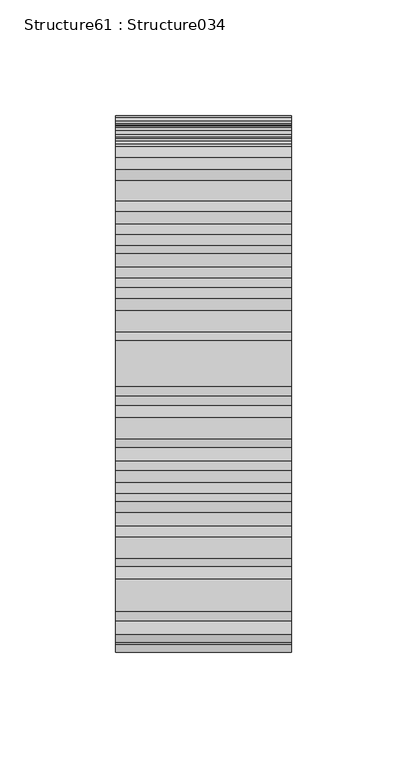
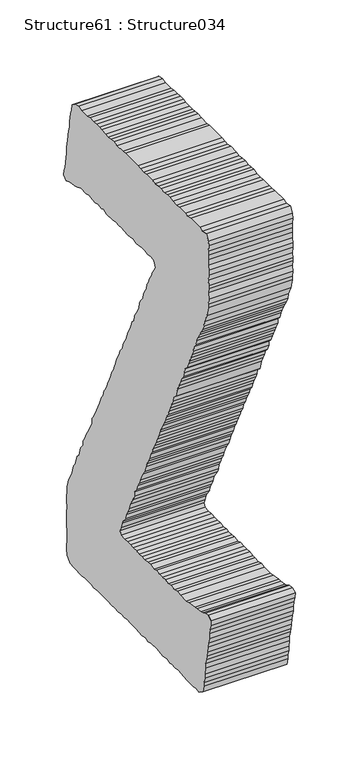
"""IFC4 building model written with IfcOpenShell, lengths in millimetres: proxy geometry, Structure61 : Structure034."""

from ifc_helpers import new_model, si_unit, frame, origin, place, context, project, spatial, polyline, outline, extrude, source, transform, mapped, element, save


def structure61_structure034_66c73dc5(model_context):
    return source(origin(), model_context, "Body", "SweptSolid", [
        extrude(outline(polyline([(280433.7807769, 3631.3410106), (280437.8789368, 3633.6821286), (280442.572405, 3633.0980525), (280446.6817971, 3630.7392839), (280450.1894625, 3629.5984101), (280456.0494781, 3628.998288), (280459.5747942, 3628.4158166), (280468.3487716, 3627.2396415), (280473.0422397, 3626.0554434), (280482.4179438, 3626.0554434), (280487.1001797, 3627.2396415), (280491.2015488, 3626.0554434), (280497.0695875, 3626.6571701), (280500.5852759, 3626.0554434), (280505.270721, 3627.2396415), (280509.952957, 3626.6571701), (280514.6464251, 3626.6571701), (280519.9127371, 3627.2396415), (280523.4284255, 3626.0554434), (280529.2884411, 3627.2396415), (280533.3978332, 3626.6571701), (280538.6641452, 3626.0554434), (280542.1894613, 3626.6571701), (280546.8652788, 3626.0554434), (280550.9730663, 3627.2396415), (280556.2506105, 3626.6571701), (280560.9232188, 3626.6571701), (280565.0245879, 3627.2396415), (280570.3085505, 3626.6571701), (280575.5828854, 3627.2396415), (280576.7510375, 3630.7392839), (280575.5828854, 3634.2822506), (280573.8162159, 3639.5405396), (280572.0655924, 3642.4833842), (280568.5402763, 3647.1575971), (280567.9658279, 3651.2589662), (280565.6166869, 3655.3587307), (280563.2739644, 3660.0682449), (280561.5153178, 3665.3265338), (280556.2506105, 3672.9435914), (280554.4823363, 3677.0449604), (280553.8982603, 3681.7271964), (280550.9730663, 3685.8285655), (280549.7888682, 3689.9540036), (280546.2812027, 3694.6298211), (280545.6971267, 3698.1294635), (280541.5973622, 3706.3289925), (280538.6641452, 3710.4560353), (280536.3214226, 3716.2887726), (280534.5724037, 3720.4158154), (280533.3978332, 3723.3313817), (280531.0470877, 3727.4311462), (280529.2884411, 3732.7167134), (280526.9553462, 3736.2163558), (280525.187072, 3740.3161203), (280522.8443495, 3744.9999608), (280520.5048361, 3749.117376), (280519.3366841, 3753.2171405), (280515.8209956, 3758.485057), (280515.2272919, 3762.5848215), (280512.2940749, 3766.684586), (280510.545056, 3771.3860772), (280508.2023335, 3775.4874463), (280505.8515879, 3779.5872107), (280504.686645, 3783.0868532), (280501.753428, 3787.2042683), (280499.9931769, 3791.8865042), (280498.8186064, 3795.4037973), (280495.895017, 3800.6717138), (280494.1363704, 3804.7730829), (280492.9682184, 3809.4729695), (280489.4509253, 3812.3901405), (280486.5193129, 3821.1737455), (280484.1765903, 3825.849563), (280482.4179438, 3830.5574726), (280480.6592973, 3834.6588416), (280477.7341033, 3838.1761347), (280475.3849623, 3843.432819), (280474.8008863, 3847.5598618), (280471.8660647, 3850.4754282), (280469.5345743, 3855.7353217), (280467.7663002, 3859.2606378), (280465.4251822, 3863.9332461), (280464.2474025, 3867.4601667), (280461.3238131, 3872.745734), (280460.7317141, 3877.4456205), (280457.8081247, 3880.9452629), (280456.630345, 3885.6210804), (280454.2988546, 3889.7208449), (280452.5321851, 3893.822214), (280449.6053865, 3897.9476522), (280447.8483446, 3901.44569), (280444.9151275, 3906.7328618), (280444.3390745, 3911.4054701), (280440.2296824, 3919.6066036), (280438.4726405, 3928.4158823), (280437.8789368, 3931.9058971), (280437.29807, 3937.1930689), (280438.4726405, 3942.4770315), (280437.29807, 3947.1496398), (280437.29807, 3950.0940891), (280437.8789368, 3954.7506513), (280437.29807, 3960.0602876), (280437.29807, 3964.7361051), (280438.4726405, 3968.8198235), (280438.4726405, 3974.1214368), (280437.8789368, 3978.8036727), (280437.8789368, 3982.8793681), (280437.29807, 3988.1633307), (280437.8789368, 3992.2614906), (280441.3978345, 3997.5486624), (280447.2642685, 3996.390138), (280451.364033, 3997.5486624), (280465.4251822, 3997.5486624), (280470.7091448, 3996.390138), (280474.2168102, 3996.9645864), (280483.5828867, 3996.9645864), (280488.2763548, 3996.390138), (280494.1363704, 3996.390138), (280498.8186064, 3997.5486624), (280502.3358994, 3997.5486624), (280507.0293676, 3996.9645864), (280512.2940749, 3997.5486624), (280516.395444, 3997.5486624), (280522.2634827, 3996.390138), (280525.7807757, 3997.5486624), (280535.1468521, 3997.5486624), (280540.4227917, 3996.390138), (280544.5321838, 3996.9645864), (280548.6319483, 3997.5486624), (280568.5402763, 3997.5486624), (280572.0655924, 3996.9645864), (280581.4332734, 3996.9645864), (280586.7188406, 3997.5486624), (280591.3930535, 3996.9645864), (280595.492818, 3996.390138), (280600.1862862, 3996.390138), (280606.0430926, 3996.9645864), (280609.5700133, 3997.5486624), (280614.2458308, 3997.5486624), (280618.9392989, 3996.9645864), (280624.2136339, 3997.5486624), (280628.8958698, 3996.390138), (280637.690707, 3996.390138), (280642.372943, 3997.5486624), (280647.6392549, 3996.390138), (280652.3327231, 3992.8375436), (280653.5072936, 3987.0048063), (280654.6834687, 3983.4794902), (280655.8484115, 3978.8036727), (280656.4421152, 3974.1214368), (280656.4421152, 3968.8198235), (280657.6070581, 3964.7361051), (280659.3657046, 3954.7506513), (280660.5418797, 3951.2606365), (280661.1243511, 3946.5511223), (280661.1243511, 3940.718385), (280661.7164502, 3937.1930689), (280662.2925032, 3931.3346579), (280663.4670737, 3926.6492128), (280665.2241156, 3922.5494483), (280665.8178193, 3917.8479571), (280661.7164502, 3914.3499193), (280657.022982, 3916.6653636), (280652.9248221, 3917.2735087), (280648.231354, 3917.8479571), (280644.1315895, 3919.0321552), (280638.2715739, 3921.3748778), (280630.0720449, 3921.3748778), (280625.9722804, 3922.5494483), (280620.1138694, 3921.3748778), (280616.0125003, 3921.3748778), (280611.3206368, 3922.5494483), (280606.0430926, 3921.3748778), (280603.1114802, 3922.5494483), (280597.8531912, 3921.3748778), (280587.8757605, 3921.3748778), (280584.3680951, 3921.9733953), (280578.509684, 3921.9733953), (280574.4083149, 3922.5494483), (280570.3085505, 3921.3748778), (280565.0245879, 3921.3748778), (280560.350375, 3921.9733953), (280556.8314773, 3922.5494483), (280551.5571423, 3921.3748778), (280547.4557732, 3921.3748778), (280542.7639097, 3922.5494483), (280538.6641452, 3922.5494483), (280533.9787001, 3921.3748778), (280528.7043651, 3922.5494483), (280524.0125016, 3921.3748778), (280521.0873076, 3916.6653636), (280523.4284255, 3912.5896682), (280525.7807757, 3909.0627475), (280527.5297946, 3904.9645876), (280530.4630116, 3900.2887701), (280532.2216582, 3895.5888836), (280534.5724037, 3892.6636896), (280535.1468521, 3887.9621984), (280538.0800692, 3883.8881076), (280540.4227917, 3879.7610648), (280541.0148908, 3875.0772243), (280543.9384802, 3871.5599312), (280546.2812027, 3867.4601667), (280547.4557732, 3862.2018778), (280549.7888682, 3857.5019912), (280553.8982603, 3850.4754282), (280555.0728308, 3845.1914656), (280557.9996294, 3842.2758992), (280559.7662989, 3837.6000817), (280561.5153178, 3833.4730389), (280564.4485348, 3828.2163546), (280566.200763, 3824.1149855), (280567.3833565, 3820.015221), (280569.718056, 3816.4883003), (280572.6416454, 3811.2043377), (280573.2337445, 3807.714323), (280576.7510375, 3803.0064134), (280577.925608, 3800.0876378), (280580.2587029, 3795.4037973), (280582.6190762, 3791.3056374), (280583.775996, 3786.6298199), (280585.5426655, 3783.0868532), (280587.2916844, 3778.4046172), (280590.2361337, 3773.7015215), (280591.9851526, 3769.0176809), (280593.7437991, 3765.5019925), (280596.0865217, 3761.418274), (280597.2610922, 3757.3185096), (280599.6038147, 3752.6170184), (280602.5274041, 3749.117376), (280603.7035792, 3743.8414364), (280606.0430926, 3740.9162424), (280607.8017391, 3736.7988273), (280609.5700133, 3732.7167134), (280613.6617547, 3723.9154578), (280616.0125003, 3719.2316172), (280618.3552229, 3714.5301261), (280620.7059685, 3711.6145597), (280621.2788123, 3706.3289925), (280623.6295579, 3702.229228), (280625.9722804, 3698.1294635), (280627.7309269, 3694.029699), (280630.6545163, 3689.9540036), (280632.9972389, 3684.6443673), (280634.7558854, 3681.7271964), (280635.3479845, 3677.0449604), (280638.8652775, 3672.3691429), (280640.023802, 3669.4262983), (280641.7888669, 3663.5598643), (280644.7140609, 3660.6250426), (280645.8886314, 3656.5429288), (280647.6392549, 3651.2589662), (280649.9900005, 3648.3161216), (280651.748647, 3643.0578326), (280653.5072936, 3638.3563415), (280655.8484115, 3634.2822506), (280657.6070581, 3630.7392839), (280659.9497806, 3622.555801), (280659.9497806, 3617.8559144), (280661.1243511, 3612.0135494), (280661.1243511, 3608.4705827), (280659.9497806, 3602.6298224), (280661.1243511, 3597.9540049), (280661.1243511, 3583.8864372), (280660.5418797, 3580.3691442), (280660.5418797, 3575.6853037), (280659.9497806, 3570.9854171), (280661.1243511, 3565.7094775), (280661.1243511, 3561.6257591), (280659.9497806, 3556.9258725), (280655.8484115, 3551.6675836), (280649.9900005, 3551.0658569), (280636.5129273, 3551.0658569), (280631.8306914, 3551.6675836), (280621.8628883, 3551.6675836), (280618.3552229, 3551.0658569), (280612.4952073, 3551.6675836), (280594.9103466, 3551.6675836), (280590.2361337, 3551.0658569), (280584.9521711, 3551.6675836), (280580.2587029, 3551.0658569), (280574.4083149, 3552.242032), (280570.3085505, 3551.0658569), (280566.200763, 3552.242032), (280560.9232188, 3551.6675836), (280552.1492414, 3551.6675836), (280547.4557732, 3551.0658569), (280542.1894613, 3551.0658569), (280536.9151263, 3552.242032), (280532.8041296, 3551.0658569), (280528.1218937, 3552.242032), (280519.3366841, 3552.242032), (280509.3704855, 3551.0658569), (280503.5120745, 3552.242032), (280498.8186064, 3551.0658569), (280495.3109409, 3552.242032), (280490.6174728, 3551.6675836), (280485.3511608, 3552.242032), (280481.2497917, 3552.242032), (280471.8660647, 3551.0658569), (280461.3238131, 3551.0658569), (280457.2240486, 3551.6675836), (280453.1146565, 3551.0658569), (280446.6817971, 3555.1848766), (280445.4959944, 3561.025637), (280444.9151275, 3565.1254015), (280443.7469755, 3569.8268927), (280443.7469755, 3573.9266571), (280443.1628994, 3579.7690221), (280442.572405, 3584.4689087), (280441.3978345, 3589.1527492), (280440.8233861, 3592.6700423), (280439.6456064, 3597.3538828), (280439.0647396, 3602.6298224), (280438.4726405, 3606.7295868), (280436.722017, 3612.0135494), (280436.722017, 3616.69739), (280435.5474465, 3621.3732075), (280434.3712714, 3626.0554434), (280433.7807769, 3631.3410106)])), frame((-59031.6926606, 0.0, 0.0), z_axis=(1.0, 0.0, 0.0), x_axis=(0.0, 1.0, 0.0)), (0.0, 0.0, 1.0), 76.2),
    ])


if __name__ == "__main__":
    model = new_model("IFC4")
    model_context = context("Model", 3, world=origin())
    ifc_project = project(units=[si_unit("LENGTHUNIT", "METRE", prefix="MILLI")], contexts=[model_context])
    site = spatial("IfcSite", under=ifc_project)
    building = spatial("IfcBuilding", under=site)
    placement = place(None, origin())
    structure61_structure034_shape = structure61_structure034_66c73dc5(model_context)
    element("IfcBuildingElementProxy", 1, Name="Structure61 : Structure034", ObjectType="Structure61 : Structure034", at=placement, inside=building, context=model_context, shape_type="MappedRepresentation", body=[
        mapped(structure61_structure034_shape, transform((0.0, 0.0, 0.0), x_axis=(1.0, 0.0, 0.0), y_axis=(0.0, 1.0, 0.0), z_axis=(0.0, 0.0, 1.0))),
    ])
    save(model, "model.ifc")

# Revit data of these elements
# Type "Structure61 : Structure034"
#   NameOverride = "Structure034"
# Element 1 (IfcBuildingElementProxy, "Structure61 : Structure034")
#   Materials on its faces: "BRUSHED ALUM. LETTERING"
# Materials
#   "BRUSHED ALUM. LETTERING": class "Unassigned", colour RGB 169 181 186, transparency 0, Cost = 0
